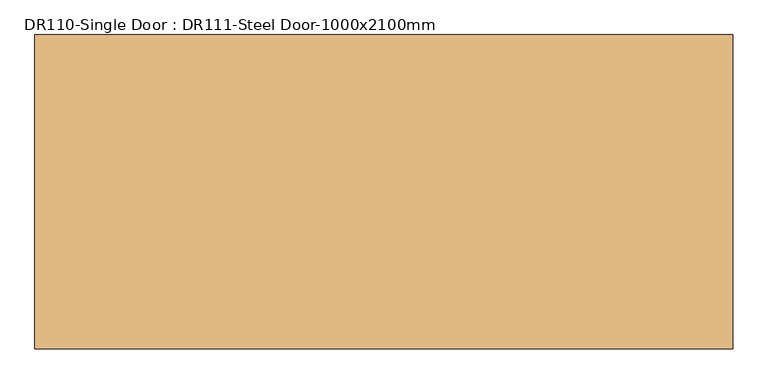
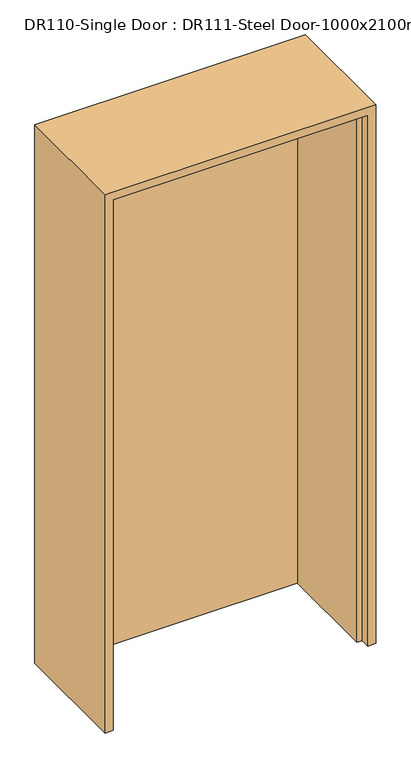
"""IFC4 building model written with IfcOpenShell, lengths in millimetres: door geometry, DR110-Single Door : DR111-Steel Door-1000x2100mm."""

from ifc_helpers import new_model, si_unit, origin, origin_with_axes, place, context, project, spatial, polyline, outline, extrude, faceted_brep, source, transform, mapped, element, save


def dr110_single_door_dr111_steel_door_1000x2100mm_e52ce95f(model_context):
    return source(origin(), model_context, "Body", "SolidModel", [
        extrude(outline(polyline([(470.0, 225.0), (470.0, 190.0), (-470.0, 190.0), (-470.0, 225.0), (470.0, 225.0)])), origin_with_axes(), (0.0, 0.0, 1.0), 2070.0),
        faceted_brep([(470.0, 225.0, 0.0), (500.0, 225.0, 0.0), (500.0, -225.0, 0.0), (470.0, -225.0, 0.0), (470.0, -190.0, 0.0), (450.0, -190.0, 0.0), (450.0, 190.0, 0.0), (470.0, 190.0, 0.0), (470.0, 225.0, 2070.0), (-470.0, 225.0, 2070.0), (-470.0, 225.0, 0.0), (-500.0, 225.0, 0.0), (-500.0, 225.0, 2100.0), (500.0, 225.0, 2100.0), (500.0, -225.0, 2100.0), (-500.0, -225.0, 2100.0), (-500.0, -225.0, 0.0), (-470.0, -225.0, 0.0), (-470.0, -225.0, 2070.0), (470.0, -225.0, 2070.0), (470.0, -190.0, 2070.0), (-470.0, -190.0, 2070.0), (-470.0, -190.0, 0.0), (-450.0, -190.0, 0.0), (-450.0, -190.0, 2050.0), (450.0, -190.0, 2050.0), (450.0, 190.0, 2050.0), (-450.0, 190.0, 2050.0), (-450.0, 190.0, 0.0), (-470.0, 190.0, 0.0), (-470.0, 190.0, 2070.0), (470.0, 190.0, 2070.0)], [[[0, 1, 2, 3, 4, 5, 6, 7]], [[1, 0, 8, 9, 10, 11, 12, 13]], [[2, 1, 13, 14]], [[3, 2, 14, 15, 16, 17, 18, 19]], [[4, 3, 19, 20]], [[5, 4, 20, 21, 22, 23, 24, 25]], [[6, 5, 25, 26]], [[7, 6, 26, 27, 28, 29, 30, 31]], [[0, 7, 31, 8]], [[9, 30, 29, 10]], [[10, 29, 28, 23, 22, 17, 16, 11]], [[15, 12, 11, 16]], [[21, 18, 17, 22]], [[27, 24, 23, 28]], [[14, 13, 12, 15]], [[20, 19, 18, 21]], [[26, 25, 24, 27]], [[8, 31, 30, 9]]]),
    ])


if __name__ == "__main__":
    model = new_model("IFC4")
    model_context = context("Model", 3, world=origin())
    ifc_project = project(units=[si_unit("LENGTHUNIT", "METRE", prefix="MILLI")], contexts=[model_context])
    site = spatial("IfcSite", under=ifc_project)
    building = spatial("IfcBuilding", under=site)
    placement = place(None, origin())
    dr110_single_door_dr111_steel_door_1000x2100mm_shape = dr110_single_door_dr111_steel_door_1000x2100mm_e52ce95f(model_context)
    element("IfcDoor", 1, ObjectType="DR110-Single Door : DR111-Steel Door-1000x2100mm", at=placement, inside=building, context=model_context, shape_type="MappedRepresentation", body=[
        mapped(dr110_single_door_dr111_steel_door_1000x2100mm_shape, transform((0.0, 0.0, 0.0), x_axis=(1.0, 0.0, 0.0), y_axis=(0.0, 1.0, 0.0), z_axis=(0.0, 0.0, 1.0))),
    ])
    save(model, "model.ifc")

# Revit data of these elements
# Type "DR110-Single Door : DR111-Steel Door-1000x2100mm"
#   Type Mark = "SD"
#   Analytic Construction = "<None>"
#   프레임 투영 외부. = 25 mm
#   프레임 투영 내부. = 25 mm
#   프레임 폭 = 75 mm
#   Height = 2100 mm
#   Width = 1000 mm
#   Define Thermal Properties by = 1
#   문 패널 = SD1 문 패널
#   문 프레임 = A04AQ098-00002_Steel Door_non FP_single
#   Function = (empty or 0)
#   Wall Closure = (empty or 0)
# Element 1 (IfcDoor, "DR110-Single Door : DR111-Steel Door-1000x2100mm")
#   Materials on its faces: "A04AQ098-00002_Steel Door_non FP_single", "SD1 문 패널"
# Materials
#   "SD1 문 패널": class "금속", colour RGB 247 247 247, transparency 0, Description = "STEEL DOOR (1000Wx2100H)"
#   "A04AQ098-00002_Steel Door_non FP_single": class "금속", colour RGB 247 247 247, transparency 0, Description = "Steel Door", W00) Work Master Code = "A04AQ098-00002", W01) Work Master_Lv1 = "Finishing Work", W02) Work Master_Lv2 = "Door & Window Work", W03) Work Master_Spec.1 = "Steel Door w/ Steel Frame", W04) Work Master_Spec.2 = "Fire Protective Rating: N/A, Single Door", W05) Work Master_Spec.3 = "w/ Hardware & Accessories", Cost = 0
